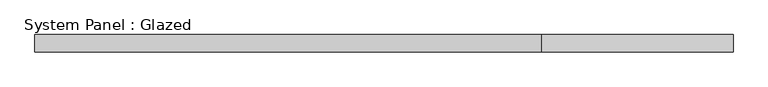
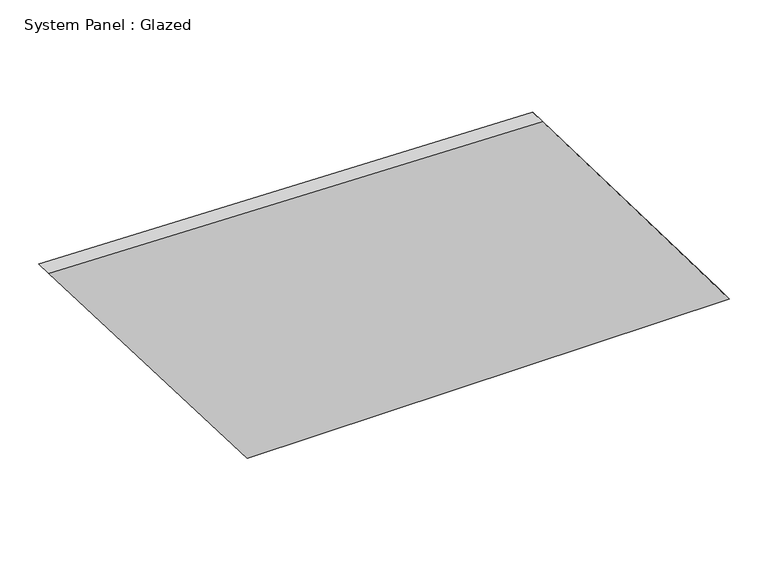
"""IFC4 building model written with IfcOpenShell, lengths in millimetres: plate geometry, System Panel : Glazed."""

from ifc_helpers import new_model, si_unit, frame, origin, place, context, project, spatial, polyline, outline, extrude, source, transform, mapped, element, save


def system_panel_glazed_7902644e(model_context):
    return source(origin(), model_context, "Body", "SweptSolid", [
        extrude(outline(polyline([(0.0, -209.6937915), (0.0, 503.6790313), (374.020594, 227.8125966), (392.0427067, -503.6790313), (0.0, -209.6937915)])), frame((0.0, -49.5, 0.0), z_axis=(0.0, 1.0, 0.0), x_axis=(0.0, 0.0, 1.0)), (0.0, 0.0, 1.0), 25.0),
    ])


if __name__ == "__main__":
    model = new_model("IFC4")
    model_context = context("Model", 3, world=origin())
    ifc_project = project(units=[si_unit("LENGTHUNIT", "METRE", prefix="MILLI")], contexts=[model_context])
    site = spatial("IfcSite", under=ifc_project)
    building = spatial("IfcBuilding", under=site)
    placement = place(None, origin())
    system_panel_glazed_shape = system_panel_glazed_7902644e(model_context)
    element("IfcPlate", 1, ObjectType="System Panel : Glazed", at=placement, inside=building, context=model_context, shape_type="MappedRepresentation", body=[
        mapped(system_panel_glazed_shape, transform((0.0, 0.0, 0.0), x_axis=(1.0, 0.0, 0.0), y_axis=(0.0, 1.0, 0.0), z_axis=(0.0, 0.0, 1.0))),
    ])
    save(model, "model.ifc")

# Revit data of these elements
# Element 1 (IfcPlate, "System Panel : Glazed")
#   Materials on its faces: "Glass, Clear Glazing"
# Materials
#   "Glass, Clear Glazing": class "Glass", colour RGB 247 249 248, transparency 0.85, Description = "Clear glazing", Cost = 0
